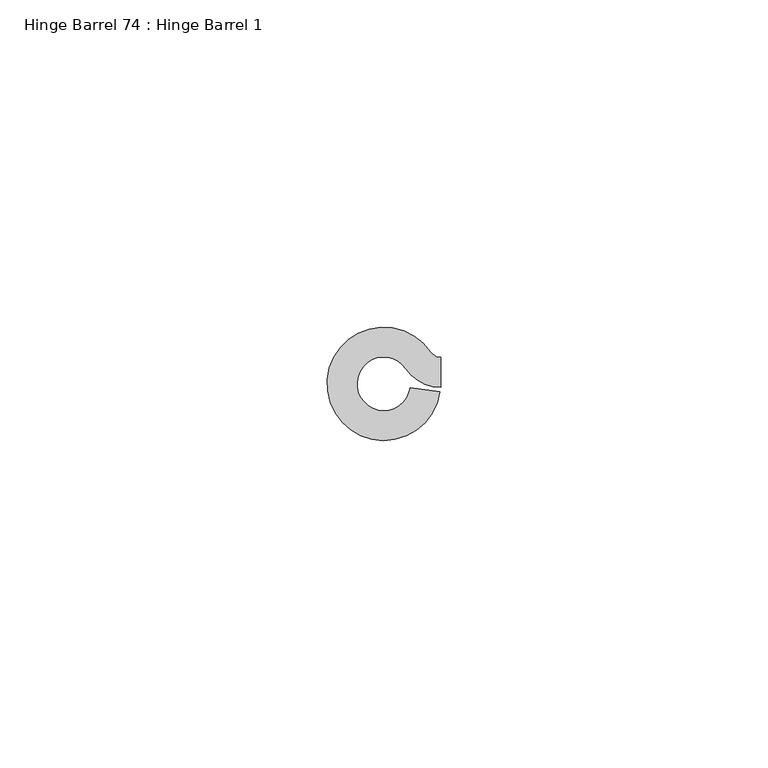
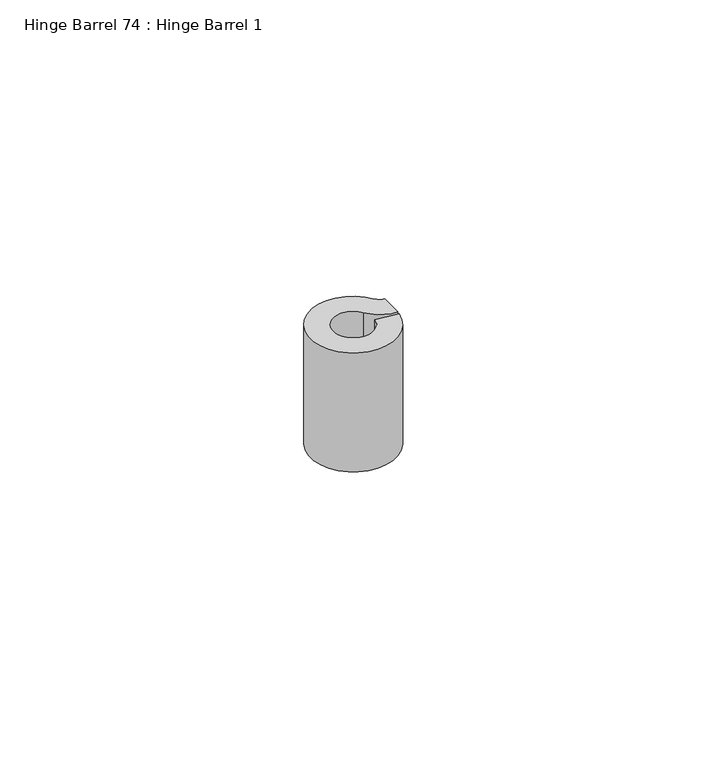
"""IFC4 building model written with IfcOpenShell, lengths in millimetres: proxy geometry, Hinge Barrel 74 : Hinge Barrel 1."""

from ifc_helpers import new_model, si_unit, point, frame, frame_2d, origin, place, context, project, spatial, polyline, circle_curve, trimmed, segment, composite_curve, outline, extrude, source, transform, mapped, element, save


def hinge_barrel_74_hinge_barrel_1_554cdc94(model_context):
    return source(origin(), model_context, "Body", "SweptSolid", [
        extrude(outline(composite_curve([segment(trimmed(circle_curve(frame_2d((587319.1320739, -531776.6049841)), 4.0894), [point((587322.5194669, -531774.3139665))], [point((587323.1821338, -531777.1708529))], True, "CARTESIAN"), True, "CONTINUOUS"), segment(polyline([(587323.1821338, -531777.1708529), (587327.7022899, -531777.8024028)]), True, "CONTINUOUS"), segment(trimmed(circle_curve(frame_2d((587319.1320739, -531776.6049841)), 8.6534625), [point((587327.7022899, -531777.8024028))], [point((587326.3000393, -531771.7570273))], False, "CARTESIAN"), True, "CONTINUOUS"), segment(trimmed(circle_curve(frame_2d((587327.8245257, -531770.7259615)), 1.8404226), [point((587326.3000393, -531771.7570273))], [point((587327.8245257, -531772.5663841))], True, "CARTESIAN"), True, "CONTINUOUS"), segment(polyline([(587327.8245257, -531772.5663841), (587327.8245257, -531777.1304466)]), True, "CONTINUOUS"), segment(trimmed(circle_curve(frame_2d((587327.8245257, -531770.7259615)), 6.4044851), [point((587327.8245257, -531777.1304466))], [point((587322.5194669, -531774.3139665))], False, "CARTESIAN"), True, "CONTINUOUS")], self_intersect=False)), frame((0.0, 0.0, 336.55), z_axis=(0.0, 0.0, 1.0), x_axis=(1.0, 0.0, 0.0)), (0.0, 0.0, 1.0), 25.4),
    ])


if __name__ == "__main__":
    model = new_model("IFC4")
    model_context = context("Model", 3, world=origin())
    ifc_project = project(units=[si_unit("LENGTHUNIT", "METRE", prefix="MILLI")], contexts=[model_context])
    site = spatial("IfcSite", under=ifc_project)
    building = spatial("IfcBuilding", under=site)
    placement = place(None, origin())
    hinge_barrel_74_hinge_barrel_1_shape = hinge_barrel_74_hinge_barrel_1_554cdc94(model_context)
    element("IfcBuildingElementProxy", 1, Name="Hinge Barrel 74 : Hinge Barrel 1", ObjectType="Hinge Barrel 74 : Hinge Barrel 1", at=placement, inside=building, context=model_context, shape_type="MappedRepresentation", body=[
        mapped(hinge_barrel_74_hinge_barrel_1_shape, transform((0.0, 0.0, 0.0), x_axis=(1.0, 0.0, 0.0), y_axis=(0.0, 1.0, 0.0), z_axis=(0.0, 0.0, 1.0))),
    ])
    save(model, "model.ifc")

# Revit data of these elements
# Element 1 (IfcBuildingElementProxy, "Hinge Barrel 74 : Hinge Barrel 1")
#   Materials on its faces: "6\"X6\" WELD-ON STL BUTT HINGE"
# Materials
#   "6\"X6\" WELD-ON STL BUTT HINGE": class "Metal", colour RGB 189 187 185, transparency 0, Description = "Carbon steel", Cost = 0
